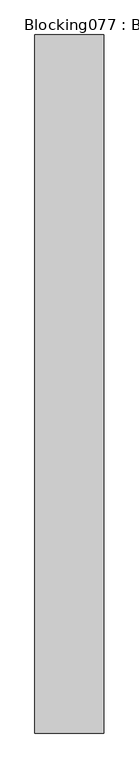
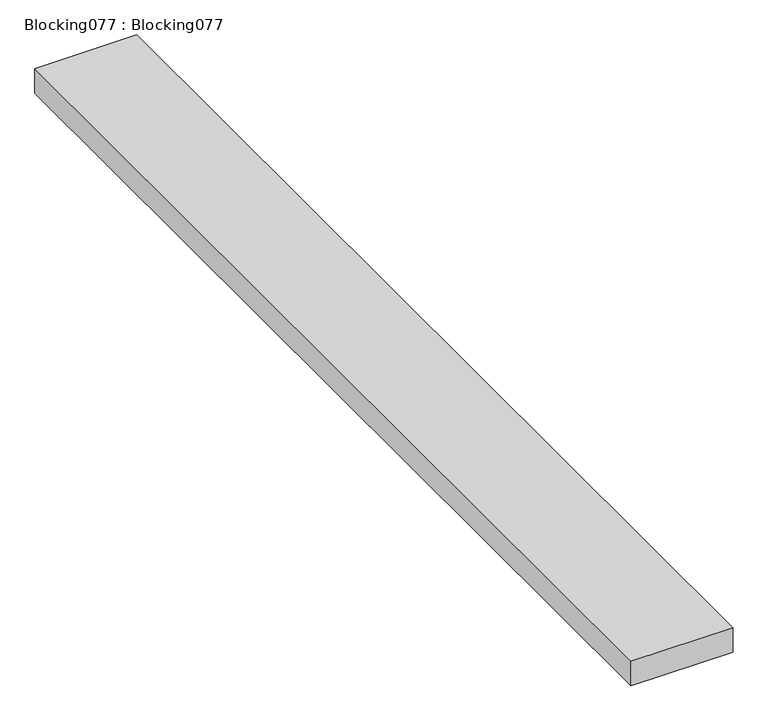
"""IFC4 building model written with IfcOpenShell, lengths in millimetres: proxy geometry, Blocking077 : Blocking077."""

from ifc_helpers import new_model, si_unit, frame, origin, place, context, project, spatial, polyline, outline, extrude, source, transform, mapped, element, save


def blocking077_blocking077_41f12090(model_context):
    return source(origin(), model_context, "Body", "SweptSolid", [
        extrude(outline(polyline([(-4797.9038825, -1052.8906574), (-4994.7538825, -1052.8906574), (-4994.7538825, 947.1093426), (-4797.9038825, 947.1093426), (-4797.9038825, -1052.8906574)])), frame((0.0, 0.0, 40182.546), z_axis=(0.0, 0.0, 1.0), x_axis=(1.0, 0.0, 0.0)), (0.0, 0.0, 1.0), 50.8),
    ])


if __name__ == "__main__":
    model = new_model("IFC4")
    model_context = context("Model", 3, world=origin())
    ifc_project = project(units=[si_unit("LENGTHUNIT", "METRE", prefix="MILLI")], contexts=[model_context])
    site = spatial("IfcSite", under=ifc_project)
    building = spatial("IfcBuilding", under=site)
    placement = place(None, origin())
    blocking077_blocking077_shape = blocking077_blocking077_41f12090(model_context)
    element("IfcBuildingElementProxy", 1, Name="Blocking077 : Blocking077", ObjectType="Blocking077 : Blocking077", at=placement, inside=building, context=model_context, shape_type="MappedRepresentation", body=[
        mapped(blocking077_blocking077_shape, transform((0.0, 0.0, 0.0), x_axis=(1.0, 0.0, 0.0), y_axis=(0.0, 1.0, 0.0), z_axis=(0.0, 0.0, 1.0))),
    ])
    save(model, "model.ifc")

# Revit data of these elements
# Type "Blocking077 : Blocking077"
#   NameOverride = "Blocking077"
# Element 1 (IfcBuildingElementProxy, "Blocking077 : Blocking077")
#   Materials on its faces: "WOOD BLOCKING AS REQUIRED"
# Materials
#   "WOOD BLOCKING AS REQUIRED": class "Unassigned", colour RGB 166 124 85, transparency 0, Cost = 0
